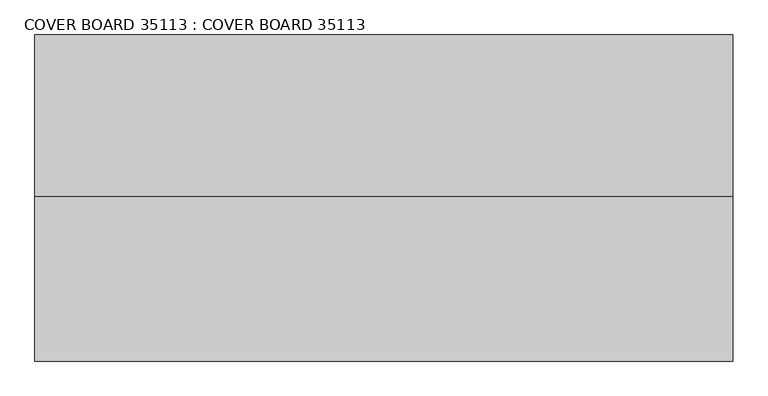
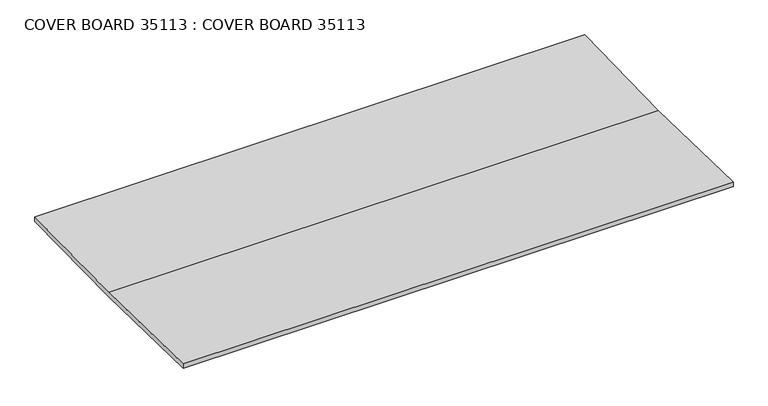
"""IFC4 building model written with IfcOpenShell, lengths in millimetres: proxy geometry, COVER BOARD 35113 : COVER BOARD 35113."""

from ifc_helpers import new_model, si_unit, frame, origin, place, context, project, spatial, polyline, outline, extrude, source, transform, mapped, element, save


def cover_board_35113_cover_board_35113_90439fdb(model_context):
    return source(origin(), model_context, "Body", "SweptSolid", [
        extrude(outline(polyline([(-4872.9612169, 40211.218553), (-4408.9401513, 40221.0164062), (-4408.9401513, 40203.6846871), (-4872.9612169, 40193.8868338), (-5343.2581759, 40203.6846871), (-5343.2581759, 40221.0164063), (-4872.9612169, 40211.218553)])), frame((12382.7678845, 0.0, 0.0), z_axis=(1.0, 0.0, 0.0), x_axis=(0.0, 1.0, 0.0)), (0.0, 0.0, 1.0), 2000.0),
    ])


if __name__ == "__main__":
    model = new_model("IFC4")
    model_context = context("Model", 3, world=origin())
    ifc_project = project(units=[si_unit("LENGTHUNIT", "METRE", prefix="MILLI")], contexts=[model_context])
    site = spatial("IfcSite", under=ifc_project)
    building = spatial("IfcBuilding", under=site)
    placement = place(None, origin())
    cover_board_35113_cover_board_35113_shape = cover_board_35113_cover_board_35113_90439fdb(model_context)
    element("IfcBuildingElementProxy", 1, Name="COVER BOARD 35113 : COVER BOARD 35113", ObjectType="COVER BOARD 35113 : COVER BOARD 35113", at=placement, inside=building, context=model_context, shape_type="MappedRepresentation", body=[
        mapped(cover_board_35113_cover_board_35113_shape, transform((0.0, 0.0, 0.0), x_axis=(1.0, 0.0, 0.0), y_axis=(0.0, 1.0, 0.0), z_axis=(0.0, 0.0, 1.0))),
    ])
    save(model, "model.ifc")

# Revit data of these elements
# Type "COVER BOARD 35113 : COVER BOARD 35113"
#   NameOverride = "COVER BOARD"
# Element 1 (IfcBuildingElementProxy, "COVER BOARD 35113 : COVER BOARD 35113")
#   Materials on its faces: "CDX PLYWOOD -  SEE STRUCTURAL DWGS"
# Materials
#   "CDX PLYWOOD -  SEE STRUCTURAL DWGS": class "Unassigned", colour RGB 138 93 50, transparency 0, Cost = 0
